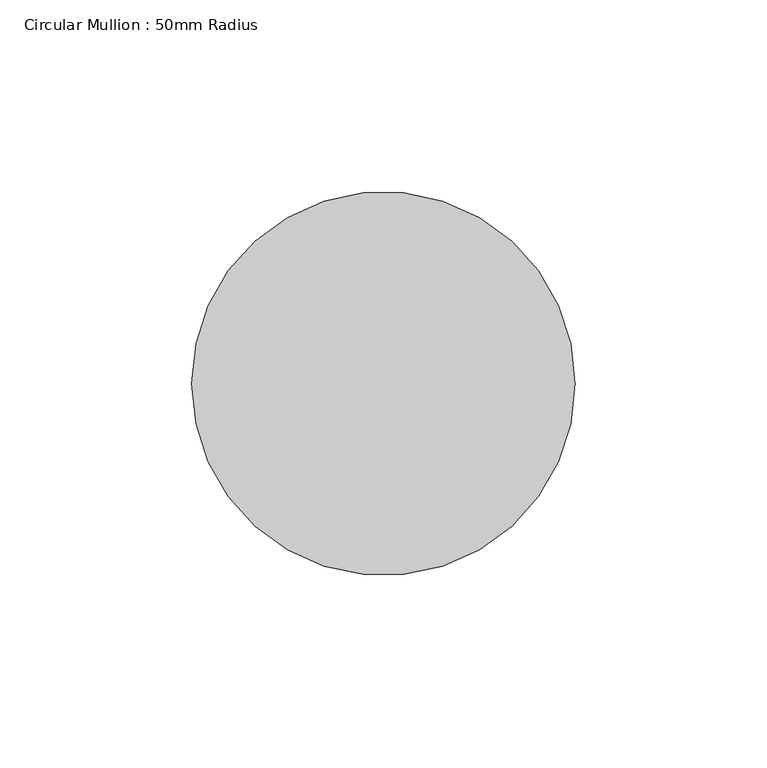
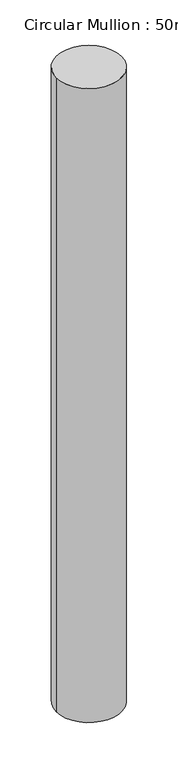
"""IFC4 building model written with IfcOpenShell, lengths in millimetres: member geometry, Circular Mullion : 50mm Radius."""

from ifc_helpers import new_model, si_unit, point, frame, origin, origin_2d, place, context, project, spatial, circle_curve, trimmed, segment, composite_curve, outline, extrude, source, transform, mapped, element, save


def circular_mullion_50mm_radius_ee00fa14(model_context):
    return source(origin(), model_context, "Body", "SweptSolid", [
        extrude(outline(composite_curve([segment(trimmed(circle_curve(origin_2d(), 50.0), [point((50.0, 0.0))], [point((-50.0, 0.0))], False, "CARTESIAN"), True, "CONTINUOUS"), segment(trimmed(circle_curve(origin_2d(), 50.0), [point((-50.0, 0.0))], [point((50.0, 0.0))], False, "CARTESIAN"), True, "CONTINUOUS")], self_intersect=False)), frame((0.0, 0.0, -1031.1502615), z_axis=(0.0, 0.0, 1.0), x_axis=(1.0, 0.0, 0.0)), (0.0, 0.0, 1.0), 1031.1502615),
    ])


if __name__ == "__main__":
    model = new_model("IFC4")
    model_context = context("Model", 3, world=origin())
    ifc_project = project(units=[si_unit("LENGTHUNIT", "METRE", prefix="MILLI")], contexts=[model_context])
    site = spatial("IfcSite", under=ifc_project)
    building = spatial("IfcBuilding", under=site)
    placement = place(None, origin())
    circular_mullion_50mm_radius_shape = circular_mullion_50mm_radius_ee00fa14(model_context)
    element("IfcMember", 1, ObjectType="Circular Mullion : 50mm Radius", at=placement, inside=building, context=model_context, shape_type="MappedRepresentation", body=[
        mapped(circular_mullion_50mm_radius_shape, transform((0.0, 0.0, 0.0), x_axis=(1.0, 0.0, 0.0), y_axis=(0.0, 1.0, 0.0), z_axis=(0.0, 0.0, 1.0))),
    ])
    save(model, "model.ifc")

# Revit data of these elements
# Type "Circular Mullion : 50mm Radius"
#   built-in parameter 1007350 = 0.164042 (stored number, unit not read)
# Element 1 (IfcMember, "Circular Mullion : 50mm Radius")
#   Materials on its faces: "Aluminium"
# Materials
#   "Aluminium": class "Metal", colour RGB 247 247 247, transparency 0, Description = "Aluminium 6061", Cost = 0
